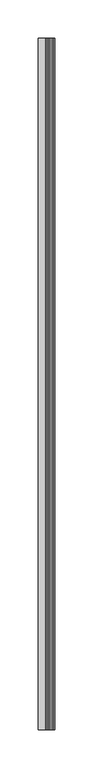
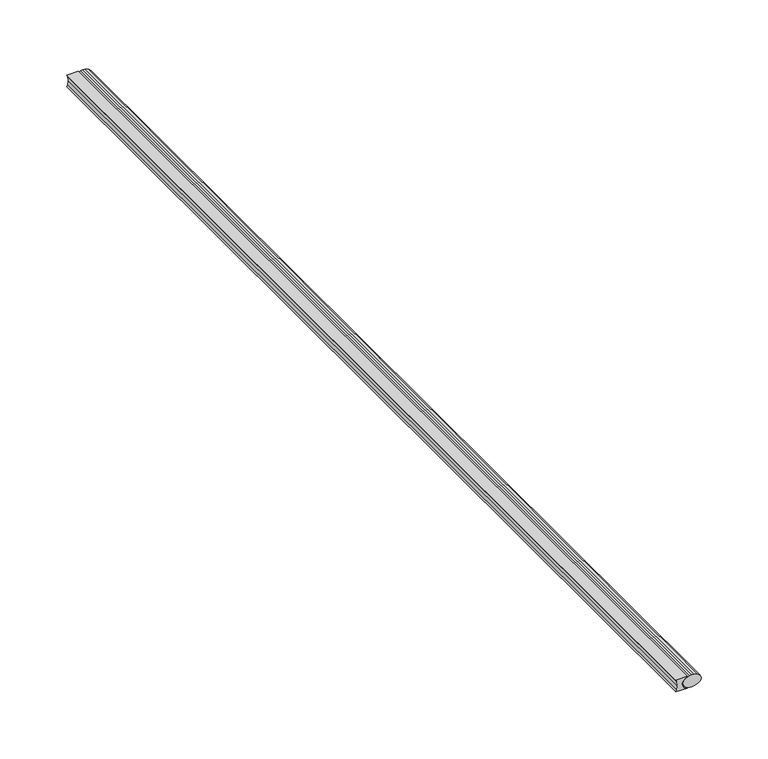
"""IFC4 building model written with IfcOpenShell, lengths in millimetres: proxy geometry, Generic Models 7:Generic Models 1:1:Generic Models 1:1 : Generic Models 7:Generic Models 1:337419:52 : Generic Models 7:Generic Models 1:1:Generic Models 1:1 : Generic Models 7:Generic Models 1:337419:306201."""

from ifc_helpers import new_model, si_unit, frame, origin, place, context, project, spatial, polyline, outline, extrude, source, transform, mapped, element, save


def generic_models_02957713(model_context):
    return source(origin(), model_context, "Body", "SweptSolid", [
        extrude(outline(polyline([(3712.6918825, 560258.0209833), (3712.6918825, 560248.1867239), (3711.0733725, 560248.8192181), (3707.3709413, 560249.3449205), (3703.66851, 560248.8192181), (3702.05, 560248.1867239), (3702.05, 560258.0209833), (3703.5294543, 560255.3509321), (3705.6098738, 560253.7182745), (3707.9657961, 560253.3784249), (3710.2286587, 560254.3845496), (3712.0444579, 560256.5792496), (3712.6918825, 560258.0209833)])), frame((0.0, -546570.8498979, 0.0), z_axis=(0.0, 1.0, 0.0), x_axis=(0.0, 0.0, 1.0)), (0.0, 0.0, 1.0), 910.0612812),
        extrude(outline(polyline([(3712.5584754, 560263.7581873), (3712.6918825, 560261.9821561), (3712.5584754, 560260.2061248), (3711.5310207, 560257.0058271), (3709.6796112, 560254.7911524), (3707.3709413, 560254.0007442), (3705.0622714, 560254.7911524), (3703.2108619, 560257.0058271), (3702.1834071, 560260.2061248), (3702.05, 560261.9821561), (3702.1834071, 560263.7581873), (3703.2108619, 560266.958485), (3705.0622714, 560269.1731597), (3707.3709413, 560269.963568), (3709.6796112, 560269.1731597), (3711.5310207, 560266.958485), (3712.5584754, 560263.7581873)])), frame((0.0, -546570.8498979, 0.0), z_axis=(0.0, 1.0, 0.0), x_axis=(0.0, 0.0, 1.0)), (0.0, 0.0, 1.0), 910.0612812),
    ])


if __name__ == "__main__":
    model = new_model("IFC4")
    model_context = context("Model", 3, world=origin())
    ifc_project = project(units=[si_unit("LENGTHUNIT", "METRE", prefix="MILLI")], contexts=[model_context])
    site = spatial("IfcSite", under=ifc_project)
    building = spatial("IfcBuilding", under=site)
    placement = place(None, origin())
    generic_models_shape = generic_models_02957713(model_context)
    element("IfcBuildingElementProxy", 1, Name="Generic Models 7:Generic Models 1:1:Generic Models 1:1 : Generic Models 7:Generic Models 1:337419:52 : Generic Models 7:Generic Models 1:1:Generic Models 1:1 : Generic Models 7:Generic Models 1:337419:306201", ObjectType="Generic Models 7:Generic Models 1:1:Generic Models 1:1 : Generic Models 7:Generic Models 1:337419:52 : Generic Models 7:Generic Models 1:1:Generic Models 1:1 : Generic Models 7:Generic Models 1:337419:306201", at=placement, inside=building, context=model_context, shape_type="MappedRepresentation", body=[
        mapped(generic_models_shape, transform((0.0, 0.0, 0.0), x_axis=(1.0, 0.0, 0.0), y_axis=(0.0, 1.0, 0.0), z_axis=(0.0, 0.0, 1.0))),
    ])
    save(model, "model.ifc")

# Revit data of these elements
# Type "Generic Models 7:Generic Models 1:1:Generic Models 1:1 : Generic Models 7:Generic Models 1:337419:52 : Generic Models 7:Generic Models 1:1:Generic Models 1:1 : Generic Models 7:Generic Models 1:337419:306201"
#   NameOverride = "Generic Models 7:Generic Models 1:1:Generic Models 1:1 : Generic Models 7:Generic Models 1:337419:306201"
#   ObjectTypeOverride = "Generic Models 1:1 : Generic Models 7:Generic Models 1:337419"
#   Reference = "Generic Models 1"
#   Tag = "306201"
# Element 1 (IfcBuildingElementProxy, "Generic Models 7:Generic Models 1:1:Generic Models 1:1 : Generic Models 7:Generic Models 1:337419:52 : Generic Models 7:Generic Models 1:1:Generic Models 1:1 : Generic Models 7:Generic Models 1:337419:306201")
#   Materials on its faces: "SEMI-RIGID EPOXY SEALANT W/ BACKROD (REMOVE TEMP. JOINT FORM)"
# Materials
#   "SEMI-RIGID EPOXY SEALANT W/ BACKROD (REMOVE TEMP. JOINT FORM)": class "Unassigned", colour RGB 120 120 120, transparency 0, Cost = 0
